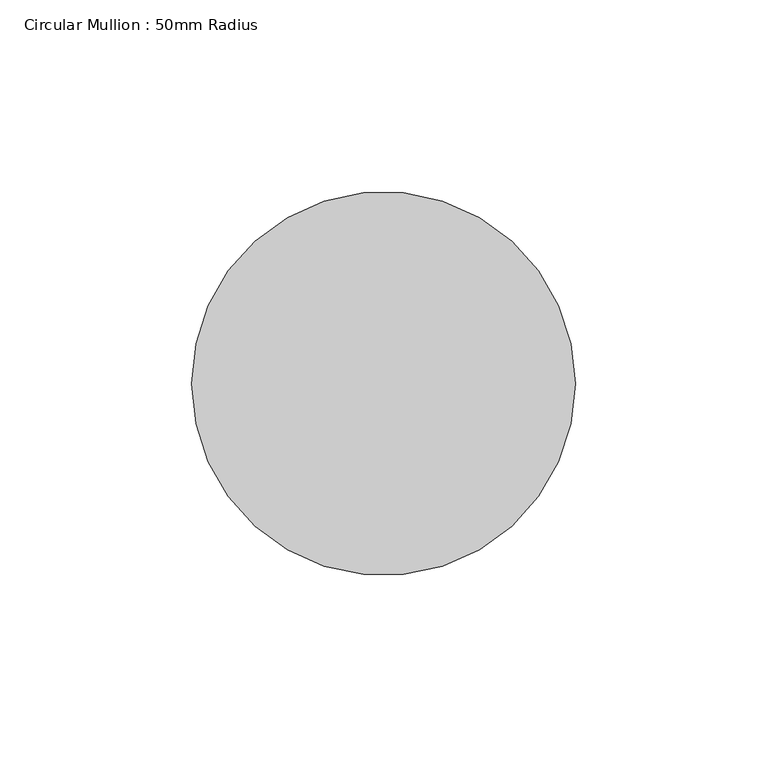
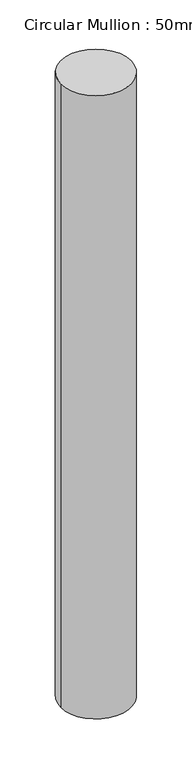
"""IFC4 building model written with IfcOpenShell, lengths in millimetres: member geometry, Circular Mullion : 50mm Radius."""

from ifc_helpers import new_model, si_unit, point, frame, origin, origin_2d, place, context, project, spatial, circle_curve, trimmed, segment, composite_curve, outline, extrude, source, transform, mapped, element, save


def circular_mullion_50mm_radius_509dadaa(model_context):
    return source(origin(), model_context, "Body", "SweptSolid", [
        extrude(outline(composite_curve([segment(trimmed(circle_curve(origin_2d(), 50.0), [point((50.0, 0.0))], [point((-50.0, 0.0))], False, "CARTESIAN"), True, "CONTINUOUS"), segment(trimmed(circle_curve(origin_2d(), 50.0), [point((-50.0, 0.0))], [point((50.0, 0.0))], False, "CARTESIAN"), True, "CONTINUOUS")], self_intersect=False)), frame((0.0, 0.0, -938.6244064), z_axis=(0.0, 0.0, 1.0), x_axis=(1.0, 0.0, 0.0)), (0.0, 0.0, 1.0), 938.6244064),
    ])


if __name__ == "__main__":
    model = new_model("IFC4")
    model_context = context("Model", 3, world=origin())
    ifc_project = project(units=[si_unit("LENGTHUNIT", "METRE", prefix="MILLI")], contexts=[model_context])
    site = spatial("IfcSite", under=ifc_project)
    building = spatial("IfcBuilding", under=site)
    placement = place(None, origin())
    circular_mullion_50mm_radius_shape = circular_mullion_50mm_radius_509dadaa(model_context)
    element("IfcMember", 1, ObjectType="Circular Mullion : 50mm Radius", at=placement, inside=building, context=model_context, shape_type="MappedRepresentation", body=[
        mapped(circular_mullion_50mm_radius_shape, transform((0.0, 0.0, 0.0), x_axis=(1.0, 0.0, 0.0), y_axis=(0.0, 1.0, 0.0), z_axis=(0.0, 0.0, 1.0))),
    ])
    save(model, "model.ifc")

# Revit data of these elements
# Type "Circular Mullion : 50mm Radius"
#   built-in parameter 1007350 = 0.164042 (stored number, unit not read)
# Element 1 (IfcMember, "Circular Mullion : 50mm Radius")
#   Materials on its faces: "Aluminium"
# Materials
#   "Aluminium": class "Metal", colour RGB 247 247 247, transparency 0, Description = "Aluminium 6061", Cost = 0
